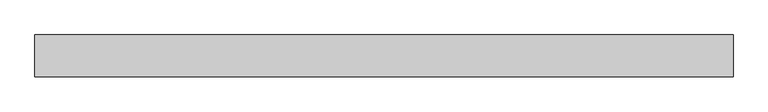
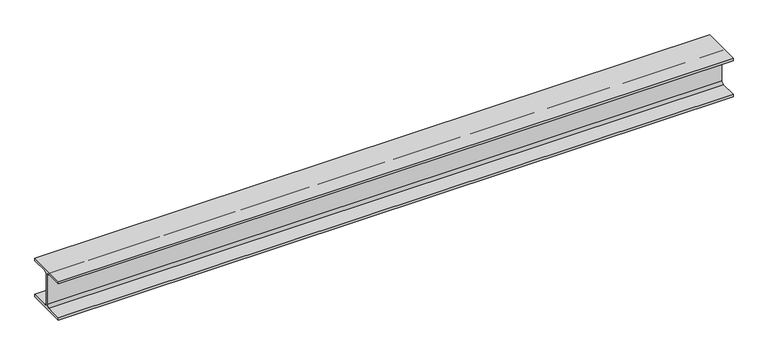
"""IFC4 building model written with IfcOpenShell, lengths in millimetres: beam geometry, 0912_Steel Framing_H-KSD3502 : H_SB_ASB_H-200x200x8x12."""

from ifc_helpers import new_model, si_unit, point, frame, frame_2d, origin, place, context, project, spatial, polyline, circle_curve, trimmed, segment, composite_curve, outline, extrude, source, transform, mapped, element, save


def beam_4e51d481(model_context):
    return source(origin(), model_context, "Body", "SweptSolid", [
        extrude(outline(composite_curve([segment(polyline([(100.0, -88.0), (100.0, -100.0), (-100.0, -100.0), (-100.0, -88.0), (-17.0, -88.0)]), True, "CONTINUOUS"), segment(trimmed(circle_curve(frame_2d((-17.0, -75.0)), 13.0), [point((-17.0, -88.0))], [point((-4.0, -75.0))], True, "CARTESIAN"), True, "CONTINUOUS"), segment(polyline([(-4.0, -75.0), (-4.0, 75.0)]), True, "CONTINUOUS"), segment(trimmed(circle_curve(frame_2d((-17.0, 75.0)), 13.0), [point((-4.0, 75.0))], [point((-17.0, 88.0))], True, "CARTESIAN"), True, "CONTINUOUS"), segment(polyline([(-17.0, 88.0), (-100.0, 88.0), (-100.0, 100.0), (100.0, 100.0), (100.0, 88.0), (17.0, 88.0)]), True, "CONTINUOUS"), segment(trimmed(circle_curve(frame_2d((17.0, 75.0)), 13.0), [point((17.0, 88.0))], [point((4.0, 75.0))], True, "CARTESIAN"), True, "CONTINUOUS"), segment(polyline([(4.0, 75.0), (4.0, -75.0)]), True, "CONTINUOUS"), segment(trimmed(circle_curve(frame_2d((17.0, -75.0)), 13.0), [point((4.0, -75.0))], [point((17.0, -88.0))], True, "CARTESIAN"), True, "CONTINUOUS"), segment(polyline([(17.0, -88.0), (100.0, -88.0)]), True, "CONTINUOUS")], self_intersect=False)), frame((-1713.7940693, 0.0, 0.0), z_axis=(1.0, 0.0, 0.0), x_axis=(0.0, 1.0, 0.0)), (0.0, 0.0, 1.0), 3322.8325842),
    ])


if __name__ == "__main__":
    model = new_model("IFC4")
    model_context = context("Model", 3, world=origin())
    ifc_project = project(units=[si_unit("LENGTHUNIT", "METRE", prefix="MILLI")], contexts=[model_context])
    site = spatial("IfcSite", under=ifc_project)
    building = spatial("IfcBuilding", under=site)
    placement = place(None, origin())
    beam_shape = beam_4e51d481(model_context)
    element("IfcBeam", 1, ObjectType="0912_Steel Framing_H-KSD3502 : H_SB_ASB_H-200x200x8x12", at=placement, inside=building, context=model_context, shape_type="MappedRepresentation", body=[
        mapped(beam_shape, transform((0.0, 0.0, 0.0), x_axis=(1.0, 0.0, 0.0), y_axis=(0.0, 1.0, 0.0), z_axis=(0.0, 0.0, 1.0))),
    ])
    save(model, "model.ifc")

# Revit data of these elements
# Type "0912_Steel Framing_H-KSD3502 : H_SB_ASB_H-200x200x8x12"
#   H_WM Code_1 = "S01AA002-00001 | Main Steel Structure Fabrication Work | Shelter/Building | Medium Steel - Standard (90KG/M>Weight≥30KG/M) | Material: (   )"
#   H_WM Code_2 = "S03AA028-00001 | Main Steel Structure Erection Work | Shelter/Building | Medium Steel (90KG/M>Weight≥30KG/M) | Material: (   )"
#   H_WM Code_3 = "S01AA010-00001 | Main Steel Structure Fabrication Work | Shelter/Building | Steel Painting/Coating | for Non-Fireproofed Steel Surface, Surface Preparation, Primer, Second & Final Coat | Material: (   )"
#   H_Q'ty Cal Type Tag = "SB-Q2"
#   Width = 20.0 cm
#   Web Thickness = 0.8 cm
#   Web Fillet = 1.3 cm
#   Warping Constant = 141000.0 cm⁶
#   W = 0
#   Torsional Moment of Inertia = 26.2485 cm⁴
#   Section Area = 63.53 cm²
#   Plastic Modulus weak axis = 244.0 cm³
#   Plastic Modulus strong axis = 525.0 cm³
#   Perimeter = 1.16 m²/m
#   Nominal Weight = 49.90 kgf/m
#   Moment of Inertia weak axis = 1600.00 cm⁴
#   Moment of Inertia strong axis = 4720.00 cm⁴
#   Height = 20.0 cm
#   Flange Thickness = 1.2 cm
#   Elastic Modulus weak axis = 160.0 cm³
#   Elastic Modulus strong axis = 472.0 cm³
#   Centroid Vertical = 10.0 cm
#   Centroid Horizontal = 10.0 cm
#   Ix = 47200000
#   Length [instance default] = 1.5240 m
#   Zx = 525000
#   b = 0.2000 m
#   h = 0.2000 m
#   r = 0.0130 m
#   s = 0.0080 m
#   t = 0.0120 m
#   A = 0.006353 m²
#   Structural Material [instance default] = Steel, 45-345
#   Assembly Code = ""
# Element 1 (IfcBeam, "0912_Steel Framing_H-KSD3502 : H_SB_ASB_H-200x200x8x12")
#   Structural Material = none
# Materials
#   "Steel, 45-345": class "Metal", colour RGB 189 187 185, transparency 0, Description = "Steel 345 MPa", Cost = 0
